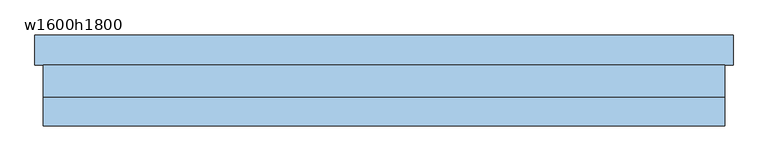
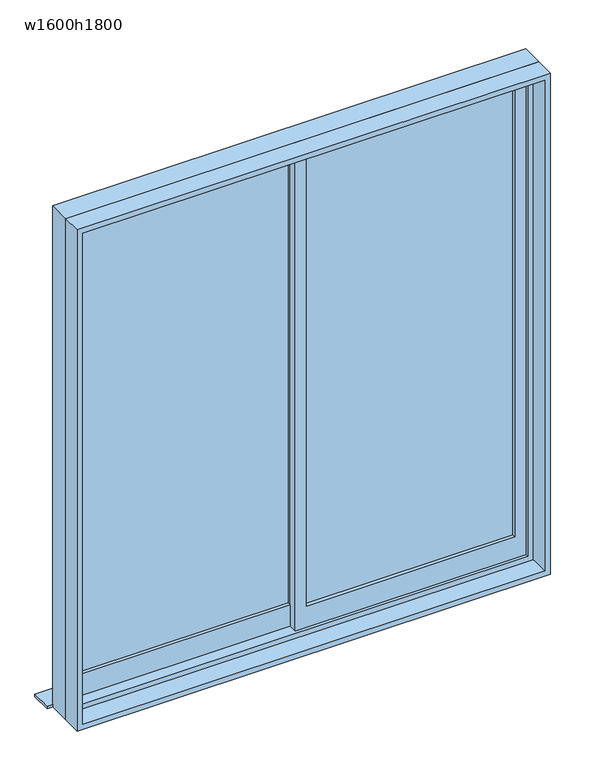
"""IFC4 building model written with IfcOpenShell, lengths in millimetres: window geometry, 引違い掃出窓_2枚 : w1600h1800."""

from ifc_helpers import new_model, si_unit, frame, origin, place, context, project, spatial, polyline, outline, extrude, source, transform, mapped, element, save


def w1600h1800_fa00a8e9(model_context):
    return source(origin(), model_context, "Body", "SweptSolid", [
        extrude(outline(polyline([(-20.0, 12.5), (-760.0, 12.5), (-760.0, 17.5), (-20.0, 17.5), (-20.0, 12.5)])), frame((0.0, 0.0, 280.0), z_axis=(0.0, 0.0, 1.0), x_axis=(1.0, 0.0, 0.0)), (0.0, 0.0, 1.0), 1680.0),
        extrude(outline(polyline([(760.0, -17.5), (20.0, -17.5), (20.0, -12.5), (760.0, -12.5), (760.0, -17.5)])), frame((0.0, 0.0, 280.0), z_axis=(0.0, 0.0, 1.0), x_axis=(1.0, 0.0, 0.0)), (0.0, 0.0, 1.0), 1680.0),
        extrude(outline(polyline([(2000.0, -20.0), (200.0, -20.0), (200.0, 800.0), (2000.0, 800.0), (2000.0, -20.0)]), holes=[polyline([(280.0, 760.0), (280.0, 20.0), (1960.0, 20.0), (1960.0, 760.0), (280.0, 760.0)])]), frame((0.0, -30.0, 0.0), z_axis=(0.0, 1.0, 0.0), x_axis=(0.0, 0.0, 1.0)), (0.0, 0.0, 1.0), 30.0),
        extrude(outline(polyline([(2000.0, -800.0), (200.0, -800.0), (200.0, 20.0), (2000.0, 20.0), (2000.0, -800.0)]), holes=[polyline([(280.0, -20.0), (280.0, -760.0), (1960.0, -760.0), (1960.0, -20.0), (280.0, -20.0)])]), frame((0.0, 0.0, 0.0), z_axis=(0.0, 1.0, 0.0), x_axis=(0.0, 0.0, 1.0)), (0.0, 0.0, 1.0), 30.0),
        extrude(outline(polyline([(860.0, 115.0), (860.0, 40.0), (-860.0, 40.0), (-860.0, 115.0), (860.0, 115.0)])), frame((0.0, 0.0, 160.0), z_axis=(0.0, 0.0, 1.0), x_axis=(1.0, 0.0, 0.0)), (0.0, 0.0, 1.0), 10.0),
        extrude(outline(polyline([(2040.0, 840.0), (2040.0, -840.0), (160.0, -840.0), (160.0, 840.0), (2040.0, 840.0)]), holes=[polyline([(180.0, -820.0), (2020.0, -820.0), (2020.0, 820.0), (180.0, 820.0), (180.0, -820.0)])]), frame((0.0, -110.0, 0.0), z_axis=(0.0, 1.0, 0.0), x_axis=(0.0, 0.0, 1.0)), (0.0, 0.0, 1.0), 70.0),
        extrude(outline(polyline([(2040.0, -840.0), (160.0, -840.0), (160.0, 840.0), (2040.0, 840.0), (2040.0, -840.0)]), holes=[polyline([(2000.0, 800.0), (200.0, 800.0), (200.0, -800.0), (2000.0, -800.0), (2000.0, 800.0)])]), frame((0.0, -40.0, 0.0), z_axis=(0.0, 1.0, 0.0), x_axis=(0.0, 0.0, 1.0)), (0.0, 0.0, 1.0), 80.0),
    ])


if __name__ == "__main__":
    model = new_model("IFC4")
    model_context = context("Model", 3, world=origin())
    ifc_project = project(units=[si_unit("LENGTHUNIT", "METRE", prefix="MILLI")], contexts=[model_context])
    site = spatial("IfcSite", under=ifc_project)
    building = spatial("IfcBuilding", under=site)
    placement = place(None, origin())
    w1600h1800_shape = w1600h1800_fa00a8e9(model_context)
    element("IfcWindow", 1, ObjectType="引違い掃出窓_2枚 : w1600h1800", at=placement, inside=building, context=model_context, shape_type="MappedRepresentation", body=[
        mapped(w1600h1800_shape, transform((0.0, 0.0, 0.0), x_axis=(1.0, 0.0, 0.0), y_axis=(0.0, 1.0, 0.0), z_axis=(0.0, 0.0, 1.0))),
    ])
    save(model, "model.ifc")

# Revit data of these elements
# Type "引違い掃出窓_2枚 : w1600h1800"
#   Type Mark = "24"
#   Operation = "ダブル パネル縦"
#   Analytic Construction = "1/8 インチ ピルキントン一重ガラス"
#   Keynote = "08520.R1"
#   Thermal Resistance (R) = 0.1491 (m²·K)/W
#   Heat Transfer Coefficient (U) = 6.7069 W/(m²·K)
#   Solar Heat Gain Coefficient = 0.86
#   Visual Light Transmittance = 0.9
#   Height = 1800 mm
#   既定の腰高 = 200 mm
#   Width = 1600 mm
#   額縁見附 = 20 mm
#   額縁ちり = 10 mm
#   サッシ見附 = 40 mm
#   サッシの幅 = 80 mm
#   Define Thermal Properties by = 1
#   サッシ額縁 [instance default] = none
#   サッシ本体 [instance default] = none
#   サッシガラス [instance default] = ガラス - 透明
#   Manufacturer = ""
#   Wall Closure = (empty or 0)
#   Model = ""
#   Type Comments = ""
#   Assembly Code = ""
# Element 1 (IfcWindow, "引違い掃出窓_2枚 : w1600h1800")
#   Materials on its faces: "ガラス - 透明"
# Materials
#   "ガラス - 透明": class "ガラス", colour RGB 0 128 255, transparency 0.9
